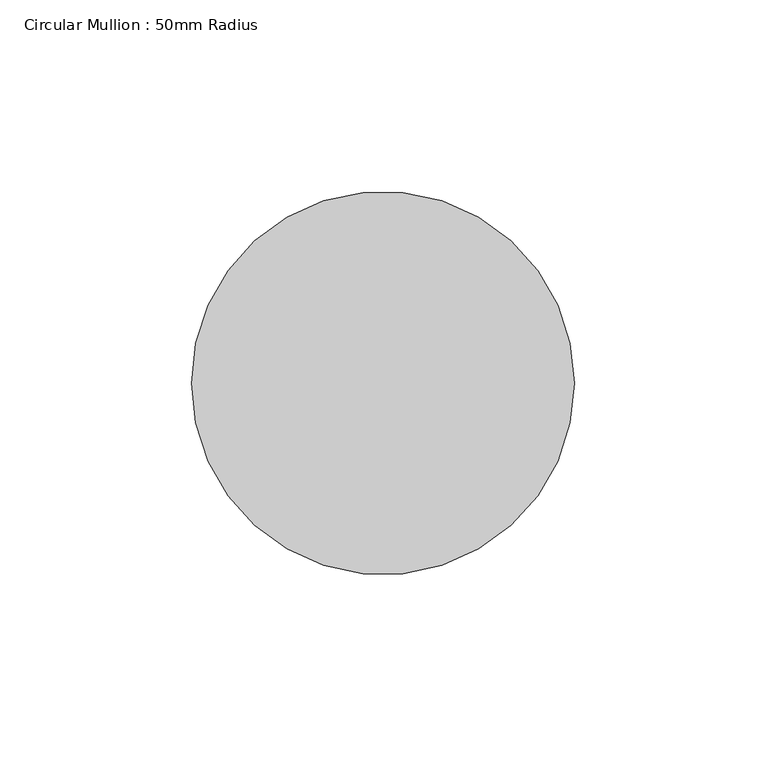
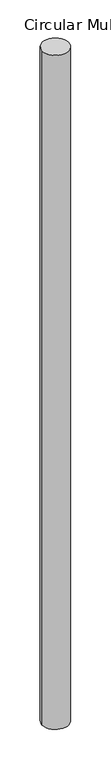
"""IFC4 building model written with IfcOpenShell, lengths in millimetres: member geometry, Circular Mullion : 50mm Radius."""

import ifcopenshell
import ifcopenshell.guid

model = None  # the IFC model being written
_history = None  # IfcOwnerHistory: only IFC2X3 demands one
_inside = {}  # id of a spatial element -> (the spatial element, [elements in it])
_under = {}  # id of a project, library or spatial element -> (it, [spatial elements below it])
_declared = {}  # id of a project -> (the project, [libraries it declares])
_typed = {}  # id of a type object -> (the type object, [elements of that type])
_made_of = {}  # id of a material, layer set ... -> (it, [elements and type objects made of it])


def new_model(schema):
    """Start an empty IFC model of exactly this schema.

    Asked for "IFC4X3", IfcOpenShell would pick the latest addendum, in which some entities
    have other attributes; the version numbers below select the first issue.
    IFC2X3 requires an IfcOwnerHistory on every rooted entity: one is made here for all.
    """
    global model, _history
    if schema == "IFC4X3":
        model = ifcopenshell.file(schema_version=(4, 3, 0, 0))
    else:
        model = ifcopenshell.file(schema=schema)
    _inside.clear()
    _under.clear()
    _declared.clear()
    _typed.clear()
    _made_of.clear()
    _history = None
    if model.schema == "IFC2X3":
        org = make("IfcOrganization", Name="unknown")
        user = make(
            "IfcPersonAndOrganization",
            ThePerson=make("IfcPerson", FamilyName="unknown"),
            TheOrganization=org,
        )
        app = make(
            "IfcApplication",
            ApplicationDeveloper=org,
            Version="unknown",
            ApplicationFullName="unknown",
            ApplicationIdentifier="unknown",
        )
        _history = make(
            "IfcOwnerHistory",
            OwningUser=user,
            OwningApplication=app,
            ChangeAction="ADDED",
            CreationDate=0,
        )
    return model


def make(cls, **values):
    """One entity of the class cls with the attributes given. An attribute that is None is left unset."""
    return model.create_entity(
        cls, **{name: value for name, value in values.items() if value is not None}
    )


def rooted(cls, **values):
    """An entity with a GlobalId (a new one), such as an element, a storey or a relation."""
    return make(cls, GlobalId=ifcopenshell.guid.new(), OwnerHistory=_history, **values)


def si_unit(unit_type, name, prefix=None):
    """IfcSIUnit, for example si_unit("LENGTHUNIT", "METRE", prefix="MILLI")."""
    return make("IfcSIUnit", UnitType=unit_type, Prefix=prefix, Name=name)


def assignment(units):
    """IfcUnitAssignment: the units of a project."""
    return None if units is None else make("IfcUnitAssignment", Units=units)


def point(xyz):
    """IfcCartesianPoint."""
    return None if xyz is None else make("IfcCartesianPoint", Coordinates=xyz)


def direction(xyz):
    """IfcDirection."""
    return None if xyz is None else make("IfcDirection", DirectionRatios=xyz)


def frame(location, z_axis=None, x_axis=None):
    """IfcAxis2Placement3D, a coordinate frame: its origin and axes. An axis left out is left unset."""
    return make(
        "IfcAxis2Placement3D",
        Location=point(location),
        Axis=direction(z_axis),
        RefDirection=direction(x_axis),
    )


def frame_2d(location, x_axis=None):
    """IfcAxis2Placement2D, a coordinate frame in the plane: its origin and x axis."""
    return make(
        "IfcAxis2Placement2D", Location=point(location), RefDirection=direction(x_axis)
    )


def origin():
    """The frame at (0, 0, 0) with its axes left unset."""
    return frame((0.0, 0.0, 0.0))


def origin_2d():
    """The frame at (0, 0) in the plane with its x axis left unset."""
    return frame_2d((0.0, 0.0))


def place(relative_to, where):
    """IfcLocalPlacement: puts the frame where relative to a parent placement (None: the world)."""
    return make(
        "IfcLocalPlacement", PlacementRelTo=relative_to, RelativePlacement=where
    )


def context(
    kind, dimensions, precision=None, world=None, true_north=None, identifier=None
):
    """IfcGeometricRepresentationContext, for example the 3D "Model" context."""
    return make(
        "IfcGeometricRepresentationContext",
        ContextIdentifier=identifier,
        ContextType=kind,
        CoordinateSpaceDimension=dimensions,
        Precision=precision,
        WorldCoordinateSystem=world,
        TrueNorth=true_north,
    )


def project(units=None, contexts=None):
    """IfcProject with its units and contexts."""
    return rooted(
        "IfcProject",
        Name="project",
        RepresentationContexts=contexts,
        UnitsInContext=assignment(units),
    )


def spatial(cls, under=None, at=None, **own):
    """A site, building, storey or space (cls), placed at a placement, below another one or the project."""
    s = rooted(cls, ObjectPlacement=at, **own)
    if under is not None:
        _under.setdefault(under.id(), (under, []))[1].append(s)
    return s


def circle_curve(where, radius):
    """IfcCircle in the frame where."""
    return make("IfcCircle", Position=where, Radius=radius)


def trimmed(basis, trim1, trim2, sense, master):
    """IfcTrimmedCurve: the piece of a basis curve between two trims."""
    return make(
        "IfcTrimmedCurve",
        BasisCurve=basis,
        Trim1=trim1,
        Trim2=trim2,
        SenseAgreement=sense,
        MasterRepresentation=master,
    )


def segment(curve, same_sense, transition):
    """IfcCompositeCurveSegment."""
    return make(
        "IfcCompositeCurveSegment",
        Transition=transition,
        SameSense=same_sense,
        ParentCurve=curve,
    )


def composite_curve(segments, self_intersect=None):
    """IfcCompositeCurve: segments joined end to end."""
    return make("IfcCompositeCurve", Segments=segments, SelfIntersect=self_intersect)


def outline(outer, holes=None, kind="AREA"):
    """IfcArbitraryClosedProfileDef: a profile drawn as a closed curve; with holes, ...WithVoids."""
    if holes is None:
        return make("IfcArbitraryClosedProfileDef", ProfileType=kind, OuterCurve=outer)
    return make(
        "IfcArbitraryProfileDefWithVoids",
        ProfileType=kind,
        OuterCurve=outer,
        InnerCurves=holes,
    )


def extrude(swept, where, along, depth):
    """IfcExtrudedAreaSolid: the profile swept, set in the frame where, extruded along a direction by depth."""
    return make(
        "IfcExtrudedAreaSolid",
        SweptArea=swept,
        Position=where,
        ExtrudedDirection=direction(along),
        Depth=depth,
    )


def shape(context_of_items, identifier, shape_type, items):
    """IfcShapeRepresentation: the items that make up one representation, for example the "Body"."""
    return make(
        "IfcShapeRepresentation",
        ContextOfItems=context_of_items,
        RepresentationIdentifier=identifier,
        RepresentationType=shape_type,
        Items=items,
    )


def source(mapping_origin, context_of_items, identifier, shape_type, items):
    """IfcRepresentationMap: a shape defined once, which mapped items show again and again."""
    return make(
        "IfcRepresentationMap",
        MappingOrigin=mapping_origin,
        MappedRepresentation=shape(context_of_items, identifier, shape_type, items),
    )


def transform(
    local_origin,
    x_axis=None,
    y_axis=None,
    z_axis=None,
    scale=None,
    scale2=None,
    scale3=None,
    uniform=True,
):
    """IfcCartesianTransformationOperator3D, or its non-uniform kind. x_axis, y_axis, z_axis: its Axis1, 2, 3."""
    if uniform:
        return make(
            "IfcCartesianTransformationOperator3D",
            Axis1=direction(x_axis),
            Axis2=direction(y_axis),
            LocalOrigin=point(local_origin),
            Scale=scale,
            Axis3=direction(z_axis),
        )
    return make(
        "IfcCartesianTransformationOperator3DnonUniform",
        Axis1=direction(x_axis),
        Axis2=direction(y_axis),
        LocalOrigin=point(local_origin),
        Scale=scale,
        Axis3=direction(z_axis),
        Scale2=scale2,
        Scale3=scale3,
    )


def mapped(mapping_source, mapping_target):
    """IfcMappedItem: shows the shape of a source again, moved by a transform."""
    return make(
        "IfcMappedItem", MappingSource=mapping_source, MappingTarget=mapping_target
    )


def made_of(thing, what):
    """Note that an element or type object is made of a material, layer set ...; save() writes the relation."""
    if what is not None:
        _made_of.setdefault(what.id(), (what, []))[1].append(thing)
    return thing


def element(
    cls,
    number,
    at=None,
    inside=None,
    cuts=None,
    type_object=None,
    material=None,
    context=None,
    identifier="Body",
    shape_type=None,
    held_by="IfcProductDefinitionShape",
    body=None,
    shapes=None,
    **own,
):
    """One element of the class cls, such as IfcWall. Its Tag is "e" and its number.

    at: its placement. inside: the storey or other place that contains it. cuts: it is an
    opening in that element (IfcRelVoidsElement). A single representation is given by context,
    identifier, shape_type and body (its items); several are given by shapes. held_by: the class
    of the entity that holds the representations. save() writes the other relations.
    """
    e = rooted(cls, Tag="e%d" % number, ObjectPlacement=at, **own)
    if body is not None:
        shapes = [shape(context, identifier, shape_type, body)]
    if shapes is not None:
        e.Representation = make(held_by, Representations=shapes)
    if inside is not None:
        _inside.setdefault(inside.id(), (inside, []))[1].append(e)
    if cuts is not None:
        rooted(
            "IfcRelVoidsElement", RelatingBuildingElement=cuts, RelatedOpeningElement=e
        )
    if type_object is not None:
        _typed.setdefault(type_object.id(), (type_object, []))[1].append(e)
    return made_of(e, material)


def aggregate(whole, parts):
    """IfcRelAggregates: a whole, such as a stair, and the parts it consists of."""
    return rooted("IfcRelAggregates", RelatingObject=whole, RelatedObjects=parts)


def save(model, path):
    """Write the relations noted so far, then the file.

    IfcRelAggregates (storeys below a building ...), IfcRelContainedInSpatialStructure (elements
    in a storey), IfcRelDefinesByType, IfcRelAssociatesMaterial and IfcRelDeclares: one each for
    every whole, place, type object, material and project.
    """
    for whole, parts in _under.values():
        aggregate(whole, parts)
    for where, things in _inside.values():
        rooted(
            "IfcRelContainedInSpatialStructure",
            RelatedElements=things,
            RelatingStructure=where,
        )
    for kind, things in _typed.values():
        rooted("IfcRelDefinesByType", RelatedObjects=things, RelatingType=kind)
    for what, things in _made_of.values():
        rooted("IfcRelAssociatesMaterial", RelatedObjects=things, RelatingMaterial=what)
    for by, libraries in _declared.values():
        rooted("IfcRelDeclares", RelatingContext=by, RelatedDefinitions=libraries)
    model.write(path)


def circular_mullion_50mm_radius_b849e295(model_context):
    return source(origin(), model_context, "Body", "SweptSolid", [
        extrude(outline(composite_curve([segment(trimmed(circle_curve(origin_2d(), 50.0), [point((50.0, 0.0))], [point((-50.0, 0.0))], False, "CARTESIAN"), True, "CONTINUOUS"), segment(trimmed(circle_curve(origin_2d(), 50.0), [point((-50.0, 0.0))], [point((50.0, 0.0))], False, "CARTESIAN"), True, "CONTINUOUS")], self_intersect=False)), frame((0.0, 0.0, -2717.4061526), z_axis=(0.0, 0.0, 1.0), x_axis=(1.0, 0.0, 0.0)), (0.0, 0.0, 1.0), 2717.4061526),
    ])


if __name__ == "__main__":
    model = new_model("IFC4")
    model_context = context("Model", 3, world=origin())
    ifc_project = project(units=[si_unit("LENGTHUNIT", "METRE", prefix="MILLI")], contexts=[model_context])
    site = spatial("IfcSite", under=ifc_project)
    building = spatial("IfcBuilding", under=site)
    placement = place(None, origin())
    circular_mullion_50mm_radius_shape = circular_mullion_50mm_radius_b849e295(model_context)
    element("IfcMember", 1, ObjectType="Circular Mullion : 50mm Radius", at=placement, inside=building, context=model_context, shape_type="MappedRepresentation", body=[
        mapped(circular_mullion_50mm_radius_shape, transform((0.0, 0.0, 0.0), x_axis=(1.0, 0.0, 0.0), y_axis=(0.0, 1.0, 0.0), z_axis=(0.0, 0.0, 1.0))),
    ])
    save(model, "model.ifc")

# Revit data of these elements
# Type "Circular Mullion : 50mm Radius"
#   built-in parameter 1007350 = 0.164042 (stored number, unit not read)
# Element 1 (IfcMember, "Circular Mullion : 50mm Radius")
#   Materials on its faces: "Aluminium"
# Materials
#   "Aluminium": class "Metal", colour RGB 247 247 247, transparency 0, Description = "Aluminium 6061", Cost = 0
